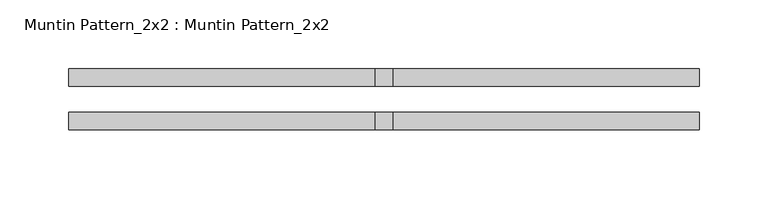
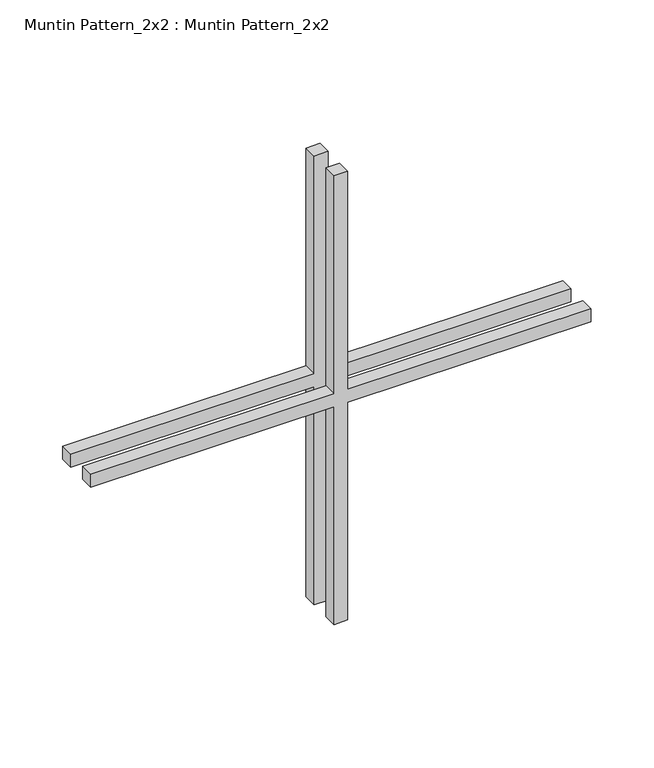
"""IFC4 building model written with IfcOpenShell, lengths in millimetres: proxy geometry, Muntin Pattern_2x2 : Muntin Pattern_2x2."""

from ifc_helpers import new_model, si_unit, frame, origin, place, context, project, spatial, polyline, outline, extrude, source, transform, mapped, element, save


def muntin_pattern_2x2_muntin_pattern_2x2_376f2fc3(model_context):
    return source(origin(), model_context, "Body", "SweptSolid", [
        extrude(outline(polyline([(223.8375, -6.35), (223.8375, -229.39375), (211.1375, -229.39375), (211.1375, -6.35), (0.0, -6.35), (0.0, 6.35), (211.1375, 6.35), (211.1375, 229.39375), (223.8375, 229.39375), (223.8375, 6.35), (434.975, 6.35), (434.975, -6.35), (223.8375, -6.35)])), frame((0.0, -22.225, 0.0), z_axis=(0.0, 1.0, 0.0), x_axis=(0.0, 0.0, 1.0)), (0.0, 0.0, 1.0), 12.7),
        extrude(outline(polyline([(223.8375, -6.35), (223.8375, -229.39375), (211.1375, -229.39375), (211.1375, -6.35), (0.0, -6.35), (0.0, 6.35), (211.1375, 6.35), (211.1375, 229.39375), (223.8375, 229.39375), (223.8375, 6.35), (434.975, 6.35), (434.975, -6.35), (223.8375, -6.35)])), frame((0.0, 9.525, 0.0), z_axis=(0.0, 1.0, 0.0), x_axis=(0.0, 0.0, 1.0)), (0.0, 0.0, 1.0), 12.7),
    ])


if __name__ == "__main__":
    model = new_model("IFC4")
    model_context = context("Model", 3, world=origin())
    ifc_project = project(units=[si_unit("LENGTHUNIT", "METRE", prefix="MILLI")], contexts=[model_context])
    site = spatial("IfcSite", under=ifc_project)
    building = spatial("IfcBuilding", under=site)
    placement = place(None, origin())
    muntin_pattern_2x2_muntin_pattern_2x2_shape = muntin_pattern_2x2_muntin_pattern_2x2_376f2fc3(model_context)
    element("IfcBuildingElementProxy", 1, Name="Muntin Pattern_2x2 : Muntin Pattern_2x2", ObjectType="Muntin Pattern_2x2 : Muntin Pattern_2x2", at=placement, inside=building, context=model_context, shape_type="MappedRepresentation", body=[
        mapped(muntin_pattern_2x2_muntin_pattern_2x2_shape, transform((0.0, 0.0, 0.0), x_axis=(1.0, 0.0, 0.0), y_axis=(0.0, 1.0, 0.0), z_axis=(0.0, 0.0, 1.0))),
    ])
    save(model, "model.ifc")

# Revit data of these elements
# Type "Muntin Pattern_2x2 : Muntin Pattern_2x2"
#   Width [instance default] = 121.92 cm
#   Thickness = 1.27 cm
#   Height [instance default] = 121.92 cm
#   Distance = 1.905 cm
#   Interior Material [instance default] = none
#   Exterior Material [instance default] = none
# Element 1 (IfcBuildingElementProxy, "Muntin Pattern_2x2 : Muntin Pattern_2x2")
#   Width = 45.8788 cm
#   Height = 43.4975 cm
#   Interior Material = Wood - Stained
#   Exterior Material = Clad - White
#   Materials on its faces: "Clad - White", "Wood - Stained"
# Materials
#   "Clad - White": class "Wood", colour RGB 242 242 238, transparency 0, Cost = 0
#   "Wood - Stained": class "Wood", colour RGB 224 178 126, transparency 0, Cost = 0
